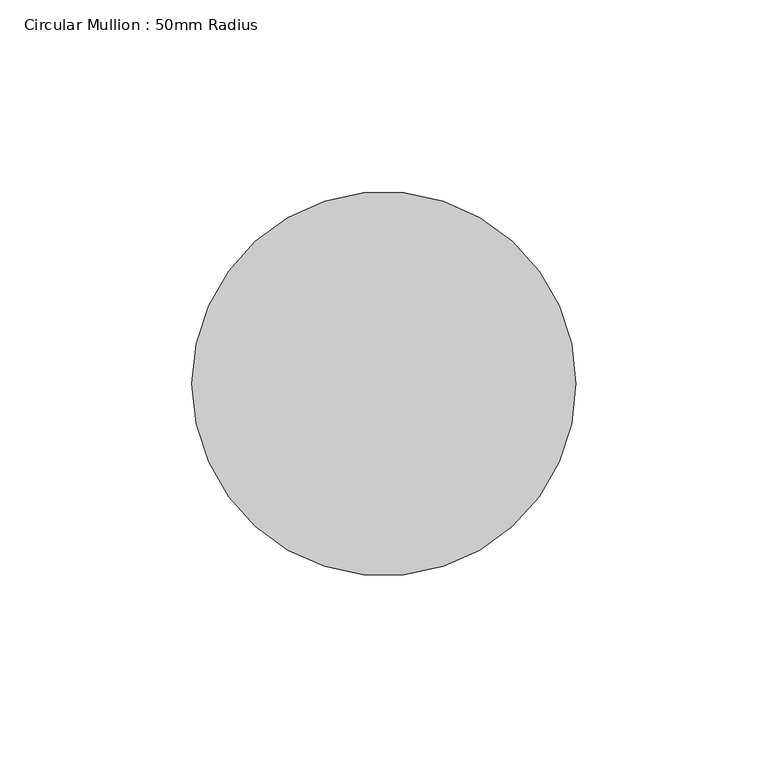
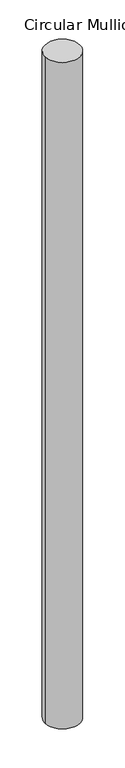
"""IFC4 building model written with IfcOpenShell, lengths in millimetres: member geometry, Circular Mullion : 50mm Radius."""

from ifc_helpers import new_model, si_unit, point, frame, frame_2d, origin, place, context, project, spatial, circle_curve, trimmed, segment, composite_curve, outline, extrude, source, transform, mapped, element, save


def circular_mullion_50mm_radius_aa9c8625(model_context):
    return source(origin(), model_context, "Body", "SweptSolid", [
        extrude(outline(composite_curve([segment(trimmed(circle_curve(frame_2d((-50.0, 0.0)), 50.0), [point((0.0, 0.0))], [point((-100.0, 0.0))], False, "CARTESIAN"), True, "CONTINUOUS"), segment(trimmed(circle_curve(frame_2d((-50.0, 0.0)), 50.0), [point((-100.0, 0.0))], [point((0.0, 0.0))], False, "CARTESIAN"), True, "CONTINUOUS")], self_intersect=False)), frame((0.0, 0.0, -2000.5090973), z_axis=(0.0, 0.0, 1.0), x_axis=(1.0, 0.0, 0.0)), (0.0, 0.0, 1.0), 2000.5090973),
    ])


if __name__ == "__main__":
    model = new_model("IFC4")
    model_context = context("Model", 3, world=origin())
    ifc_project = project(units=[si_unit("LENGTHUNIT", "METRE", prefix="MILLI")], contexts=[model_context])
    site = spatial("IfcSite", under=ifc_project)
    building = spatial("IfcBuilding", under=site)
    placement = place(None, origin())
    circular_mullion_50mm_radius_shape = circular_mullion_50mm_radius_aa9c8625(model_context)
    element("IfcMember", 1, ObjectType="Circular Mullion : 50mm Radius", at=placement, inside=building, context=model_context, shape_type="MappedRepresentation", body=[
        mapped(circular_mullion_50mm_radius_shape, transform((0.0, 0.0, 0.0), x_axis=(1.0, 0.0, 0.0), y_axis=(0.0, 1.0, 0.0), z_axis=(0.0, 0.0, 1.0))),
    ])
    save(model, "model.ifc")

# Revit data of these elements
# Type "Circular Mullion : 50mm Radius"
#   built-in parameter 1007350 = 0.164042 (stored number, unit not read)
# Element 1 (IfcMember, "Circular Mullion : 50mm Radius")
#   Materials on its faces: "Aluminium"
# Materials
#   "Aluminium": class "Metal", colour RGB 247 247 247, transparency 0, Description = "Aluminium 6061", Cost = 0
